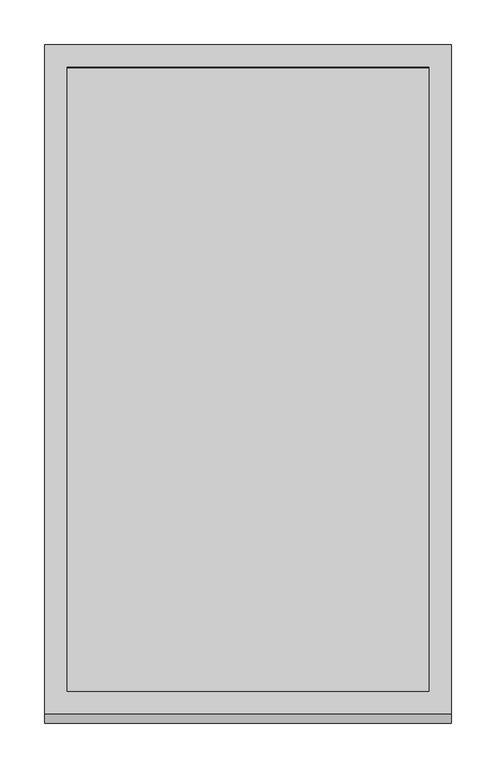
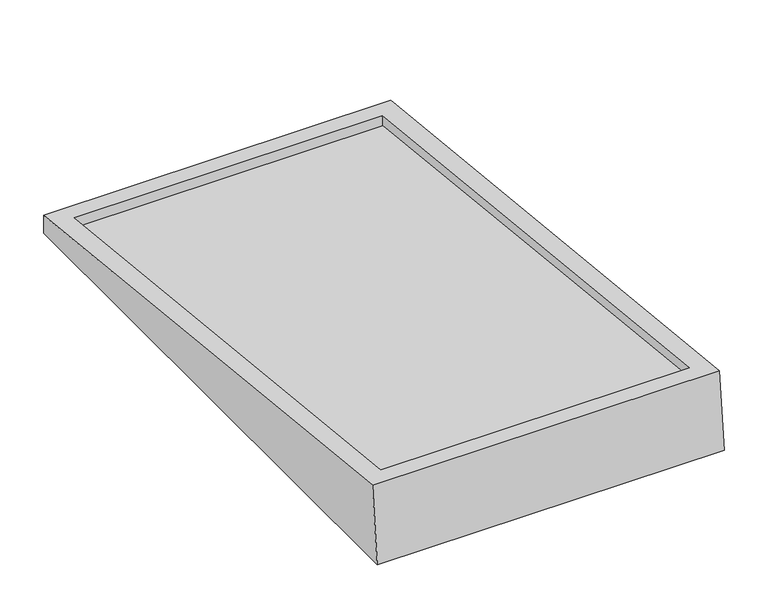
"""IFC4 building model written with IfcOpenShell, lengths in millimetres: proxy geometry, Bradley-Washroom_Accessories-Mirrors-740_Custom : Bradley-Washroom_Accessories-Mirrors-740_Custom."""

from ifc_helpers import new_model, si_unit, origin, place, context, project, spatial, faceted_brep, source, transform, mapped, element, save


def specialty_equipment_28a0cf3e(model_context):
    return source(origin(), model_context, "Body", "Brep", [
        faceted_brep([(228.6, 381.0, 0.0), (228.6, 381.0, 25.4), (228.6, -370.0337574, 104.3368287), (228.6, -381.0, 0.0), (-228.6, 381.0, 0.0), (-228.6, -381.0, 0.0), (-228.6, -370.0337574, 104.3368287), (-228.6, 381.0, 25.4), (-203.2, 355.7391439, 28.055023), (203.2, 355.7391439, 28.055023), (203.2, -344.7729013, 101.6818058), (-203.2, -344.7729013, 101.6818058), (-203.2, 354.4116324, 15.4245949), (-203.2, -346.1004127, 89.0513777), (203.2, -346.1004127, 89.0513777), (203.2, 354.4116324, 15.4245949)], [[[0, 1, 2, 3]], [[4, 5, 6, 7]], [[3, 5, 4, 0]], [[2, 6, 5, 3]], [[1, 7, 6, 2], [8, 9, 10, 11]], [[0, 4, 7, 1]], [[12, 13, 14, 15]], [[12, 8, 11, 13]], [[13, 11, 10, 14]], [[14, 10, 9, 15]], [[15, 9, 8, 12]]]),
    ])


if __name__ == "__main__":
    model = new_model("IFC4")
    model_context = context("Model", 3, world=origin())
    ifc_project = project(units=[si_unit("LENGTHUNIT", "METRE", prefix="MILLI")], contexts=[model_context])
    site = spatial("IfcSite", under=ifc_project)
    building = spatial("IfcBuilding", under=site)
    placement = place(None, origin())
    specialty_equipment_shape = specialty_equipment_28a0cf3e(model_context)
    element("IfcBuildingElementProxy", 1, Name="Bradley-Washroom_Accessories-Mirrors-740_Custom : Bradley-Washroom_Accessories-Mirrors-740_Custom", ObjectType="Bradley-Washroom_Accessories-Mirrors-740_Custom : Bradley-Washroom_Accessories-Mirrors-740_Custom", at=placement, inside=building, context=model_context, shape_type="MappedRepresentation", body=[
        mapped(specialty_equipment_shape, transform((0.0, 0.0, 0.0), x_axis=(1.0, 0.0, 0.0), y_axis=(0.0, 1.0, 0.0), z_axis=(0.0, 0.0, 1.0))),
    ])
    save(model, "model.ifc")

# Revit data of these elements
# Type "Bradley-Washroom_Accessories-Mirrors-740_Custom : Bradley-Washroom_Accessories-Mirrors-740_Custom"
#   Warranty Information = "Complete unit, excepting mirrors warranted for one year.\r\n Stainless steel mirror frames for fifteen years.\r\n Plate glass mirrors for fifteen years.\r\n This warranty does not cover installation or any other labor charges and does not apply to any units,\r\n which have been damaged by accident, abuse, improper installation, improper maintenance, or altered in any way."
#   Version = "1.0"
#   URL = "http://www.bradleycorp.com/"
#   Type Comments = "ERROR - If you are able to see this message you haven't loaded this  family correctly."
#   OmniClass Title = "Mirrors"
#   OmniClass Code = "23.40.95.17.17"
#   Modeling Code = ""
#   Model = "740-A"
#   MasterFormat Title = "Commercial Toilet Accessories"
#   MasterFormat Number = "10 28 13. 13"
#   Manufacturer = "Bradley Corporation"
#   Industry Standards = "ASTM C 1036"
#   Fire Rating = "n/a"
#   Dimensional Limits [instance default] = "Either Width or Hight must be over 25\""
#   Description = "ERROR - If you are able to see this message you haven't loaded this  family correctly."
#   Copyright = "This Model Data is Property of Bradley Corporation"
#   Buy American Act = "Yes"
#   Assembly Code = "C1030900"
#   ADA Compliant = "Yes"
#   Width [instance default] = 457.2 mm
#   Total Width [instance default] = 457.2 mm
#   Total Height [instance default] = 762 mm
#   Total Depth [instance default] = 105.051 mm
#   Height [instance default] = 762 mm
#   Depth [instance default] = 105.051 mm
#   Default Elevation = 1016 mm
#   Reflective Material = Glass - Bradley Corp - BradEX - Polished Float Mirror
#   Frame Material = Bradley Corp Stainless Steel - Satin
# Element 1 (IfcBuildingElementProxy, "Bradley-Washroom_Accessories-Mirrors-740_Custom : Bradley-Washroom_Accessories-Mirrors-740_Custom")
#   Materials on its faces: "Bradley Corp Stainless Steel - Satin"
# Materials
#   "Glass - Bradley Corp - BradEX - Polished Float Mirror": class "Glass", colour RGB 220 232 220, transparency 0, Manufacturer = "Bradley Corporation", URL = "www.bradleycorp.com", Description = "Stainless Steel - Satin Finish", Cost = 0
#   "Bradley Corp Stainless Steel - Satin": class "Metal", colour RGB 189 187 185, transparency 0, Manufacturer = "Bradley Corporation", URL = "www.bradleycorp.com", Description = "Stainless Steel - Satin Finish", Cost = 0
